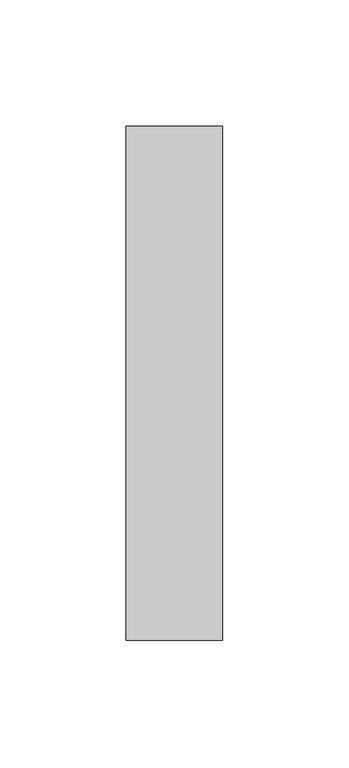
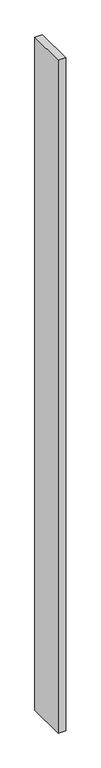
"""IFC4 building model written with IfcOpenShell, lengths in millimetres: proxy geometry, Lower profile:Lower profile:1:Lower profile:1 : Lower profile:Lower profile:300380:301093:Lower profile:1:Lower profile:1 : Lower profile:Lower profile:300380:301093 : Lower profile:Lower profile:1:Lower profile:1 : Lower profile:Lower profile:300380:301093:1 : Lower profile:Lower profile:1:Lower profile:1 : Lower profile:Lower profile:300380:301093:Lower profile:1:Lower profile:1 : Lower profile:Lower profile:300380:301093 : Lower profile:Lower profile:1:Lower profile:1 : Lower profile:Lower profile:300380:301093:300247."""

from ifc_helpers import new_model, si_unit, frame, origin, place, context, project, spatial, polyline, outline, extrude, source, transform, mapped, element, save


def generic_models_f5dbdf07(model_context):
    return source(origin(), model_context, "Body", "SweptSolid", [
        extrude(outline(polyline([(593776.1867239, -578797.4913841), (593776.1867239, -579000.6913841), (593738.0867239, -579000.6913841), (593738.0867239, -578797.4913841), (593776.1867239, -578797.4913841)])), frame((0.0, 0.0, 44.45), z_axis=(0.0, 0.0, 1.0), x_axis=(1.0, 0.0, 0.0)), (0.0, 0.0, 1.0), 3590.2304687),
    ])


if __name__ == "__main__":
    model = new_model("IFC4")
    model_context = context("Model", 3, world=origin())
    ifc_project = project(units=[si_unit("LENGTHUNIT", "METRE", prefix="MILLI")], contexts=[model_context])
    site = spatial("IfcSite", under=ifc_project)
    building = spatial("IfcBuilding", under=site)
    placement = place(None, origin())
    generic_models_shape = generic_models_f5dbdf07(model_context)
    element("IfcBuildingElementProxy", 1, Name="Lower profile:Lower profile:1:Lower profile:1 : Lower profile:Lower profile:300380:301093:Lower profile:1:Lower profile:1 : Lower profile:Lower profile:300380:301093 : Lower profile:Lower profile:1:Lower profile:1 : Lower profile:Lower profile:300380:301093:1 : Lower profile:Lower profile:1:Lower profile:1 : Lower profile:Lower profile:300380:301093:Lower profile:1:Lower profile:1 : Lower profile:Lower profile:300380:301093 : Lower profile:Lower profile:1:Lower profile:1 : Lower profile:Lower profile:300380:301093:300247", ObjectType="Lower profile:Lower profile:1:Lower profile:1 : Lower profile:Lower profile:300380:301093:Lower profile:1:Lower profile:1 : Lower profile:Lower profile:300380:301093 : Lower profile:Lower profile:1:Lower profile:1 : Lower profile:Lower profile:300380:301093:1 : Lower profile:Lower profile:1:Lower profile:1 : Lower profile:Lower profile:300380:301093:Lower profile:1:Lower profile:1 : Lower profile:Lower profile:300380:301093 : Lower profile:Lower profile:1:Lower profile:1 : Lower profile:Lower profile:300380:301093:300247", at=placement, inside=building, context=model_context, shape_type="MappedRepresentation", body=[
        mapped(generic_models_shape, transform((0.0, 0.0, 0.0), x_axis=(1.0, 0.0, 0.0), y_axis=(0.0, 1.0, 0.0), z_axis=(0.0, 0.0, 1.0))),
    ])
    save(model, "model.ifc")

# Revit data of these elements
# Type "Lower profile:Lower profile:1:Lower profile:1 : Lower profile:Lower profile:300380:301093:Lower profile:1:Lower profile:1 : Lower profile:Lower profile:300380:301093 : Lower profile:Lower profile:1:Lower profile:1 : Lower profile:Lower profile:300380:301093:1 : Lower profile:Lower profile:1:Lower profile:1 : Lower profile:Lower profile:300380:301093:Lower profile:1:Lower profile:1 : Lower profile:Lower profile:300380:301093 : Lower profile:Lower profile:1:Lower profile:1 : Lower profile:Lower profile:300380:301093:300247"
#   NameOverride = "Lower profile:Lower profile:1:Lower profile:1 : Lower profile:Lower profile:300380:301093:Lower profile:1:Lower profile:1 : Lower profile:Lower profile:300380:301093 : Lower profile:Lower profile:1:Lower profile:1 : Lower profile:Lower profile:300380:301093:300247"
#   ObjectTypeOverride = "Lower profile:1:Lower profile:1 : Lower profile:Lower profile:300380:301093 : Lower profile:Lower profile:1:Lower profile:1 : Lower profile:Lower profile:300380:301093"
#   Reference = "Lower profile"
#   Tag = "300247"
# Element 1 (IfcBuildingElementProxy, "Lower profile:Lower profile:1:Lower profile:1 : Lower profile:Lower profile:300380:301093:Lower profile:1:Lower profile:1 : Lower profile:Lower profile:300380:301093 : Lower profile:Lower profile:1:Lower profile:1 : Lower profile:Lower profile:300380:301093:1 : Lower profile:Lower profile:1:Lower profile:1 : Lower profile:Lower profile:300380:301093:Lower profile:1:Lower profile:1 : Lower profile:Lower profile:300380:301093 : Lower profile:Lower profile:1:Lower profile:1 : Lower profile:Lower profile:300380:301093:300247")
#   Materials on its faces: "BLOCKING - SIZE AS NEC."
# Materials
#   "BLOCKING - SIZE AS NEC.": class "Wood", colour RGB 144 113 62, transparency 0, Description = "Pinus Echinata", Cost = 0
